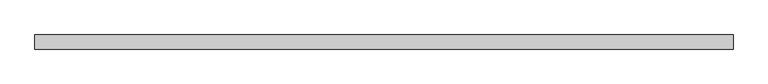
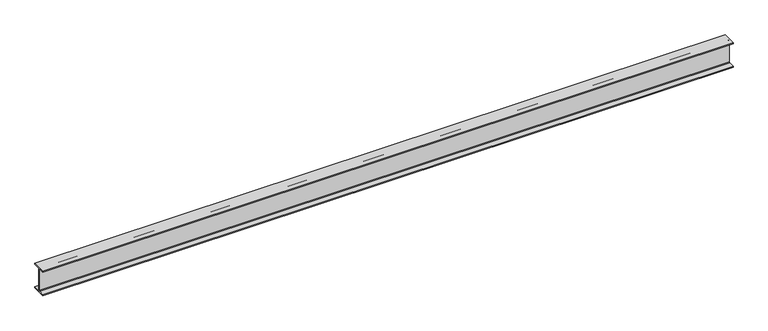
"""IFC4 building model written with IfcOpenShell, lengths in millimetres: beam geometry, Old_Steel Beam_H-KSD3502 : H_SB_ASB_H-340×250x9x14."""

from ifc_helpers import new_model, si_unit, point, frame, frame_2d, origin, place, context, project, spatial, polyline, circle_curve, trimmed, segment, composite_curve, outline, extrude, source, transform, mapped, element, save


def beam_dd981bdd(model_context):
    return source(origin(), model_context, "Body", "SweptSolid", [
        extrude(outline(composite_curve([segment(polyline([(82.5, -141.5), (82.5, -151.7), (-82.5, -151.7), (-82.5, -141.5), (-11.9, -141.5)]), True, "CONTINUOUS"), segment(trimmed(circle_curve(frame_2d((-11.9, -132.6)), 8.9), [point((-11.9, -141.5))], [point((-3.0, -132.6))], True, "CARTESIAN"), True, "CONTINUOUS"), segment(polyline([(-3.0, -132.6), (-3.0, 132.6)]), True, "CONTINUOUS"), segment(trimmed(circle_curve(frame_2d((-11.9, 132.6)), 8.9), [point((-3.0, 132.6))], [point((-11.9, 141.5))], True, "CARTESIAN"), True, "CONTINUOUS"), segment(polyline([(-11.9, 141.5), (-82.5, 141.5), (-82.5, 151.7), (82.5, 151.7), (82.5, 141.5), (11.9, 141.5)]), True, "CONTINUOUS"), segment(trimmed(circle_curve(frame_2d((11.9, 132.6)), 8.9), [point((11.9, 141.5))], [point((3.0, 132.6))], True, "CARTESIAN"), True, "CONTINUOUS"), segment(polyline([(3.0, 132.6), (3.0, -132.6)]), True, "CONTINUOUS"), segment(trimmed(circle_curve(frame_2d((11.9, -132.6)), 8.9), [point((3.0, -132.6))], [point((11.9, -141.5))], True, "CARTESIAN"), True, "CONTINUOUS"), segment(polyline([(11.9, -141.5), (82.5, -141.5)]), True, "CONTINUOUS")], self_intersect=False)), frame((-4087.3, 0.0, 0.0), z_axis=(1.0, 0.0, 0.0), x_axis=(0.0, 1.0, 0.0)), (0.0, 0.0, 1.0), 8174.6),
    ])


if __name__ == "__main__":
    model = new_model("IFC4")
    model_context = context("Model", 3, world=origin())
    ifc_project = project(units=[si_unit("LENGTHUNIT", "METRE", prefix="MILLI")], contexts=[model_context])
    site = spatial("IfcSite", under=ifc_project)
    building = spatial("IfcBuilding", under=site)
    placement = place(None, origin())
    beam_shape = beam_dd981bdd(model_context)
    element("IfcBeam", 1, ObjectType="Old_Steel Beam_H-KSD3502 : H_SB_ASB_H-340×250x9x14", at=placement, inside=building, context=model_context, shape_type="MappedRepresentation", body=[
        mapped(beam_shape, transform((0.0, 0.0, 0.0), x_axis=(1.0, 0.0, 0.0), y_axis=(0.0, 1.0, 0.0), z_axis=(0.0, 0.0, 1.0))),
    ])
    save(model, "model.ifc")

# Revit data of these elements
# Type "Old_Steel Beam_H-KSD3502 : H_SB_ASB_H-340×250x9x14"
#   Width = 25.0 cm
#   Web Thickness = 0.9 cm
#   Web Fillet = 2.0 cm
#   Warping Constant = 968661.0 cm⁶
#   Torsional Moment of Inertia = 53.6551 cm⁴
#   Torsional Modulus = 1.0 cm³
#   Section Area = 101.5 cm²
#   Plastic Modulus weak axis = 447.0 cm³
#   Plastic Modulus strong axis = 1410.0 cm³
#   Perimeter = 1.63 m²/m
#   Nominal Weight = 79.70 kgf/m
#   Moment of Inertia weak axis = 3650.00 cm⁴
#   Moment of Inertia strong axis = 21700.00 cm⁴
#   Height = 34.0 cm
#   Flange Thickness = 1.4 cm
#   Elastic Modulus weak axis = 292.0 cm³
#   Elastic Modulus strong axis = 1280.0 cm³
#   Centroid Vertical = 17.0 cm
#   Centroid Horizontal = 12.5 cm
#   Length [instance default] = 1.5240 m
#   Structural Material [instance default] = Steel, 45-345
#   Assembly Code = ""
# Element 1 (IfcBeam, "Old_Steel Beam_H-KSD3502 : H_SB_ASB_H-340×250x9x14")
#   Structural Material = none
# Materials
#   "Steel, 45-345": class "Metal", colour RGB 189 187 185, transparency 0, Description = "Steel 345 MPa", Cost = 0
